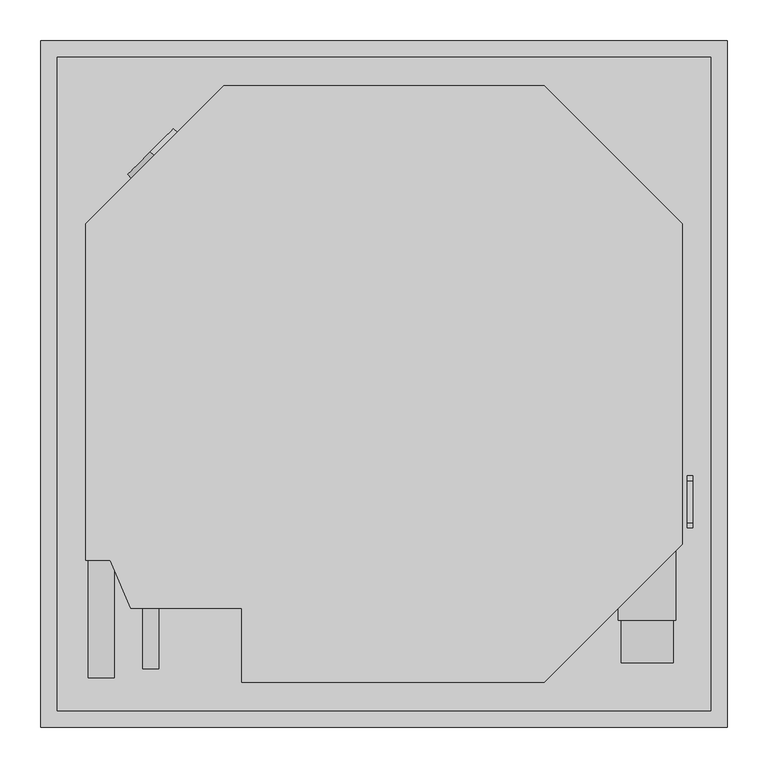
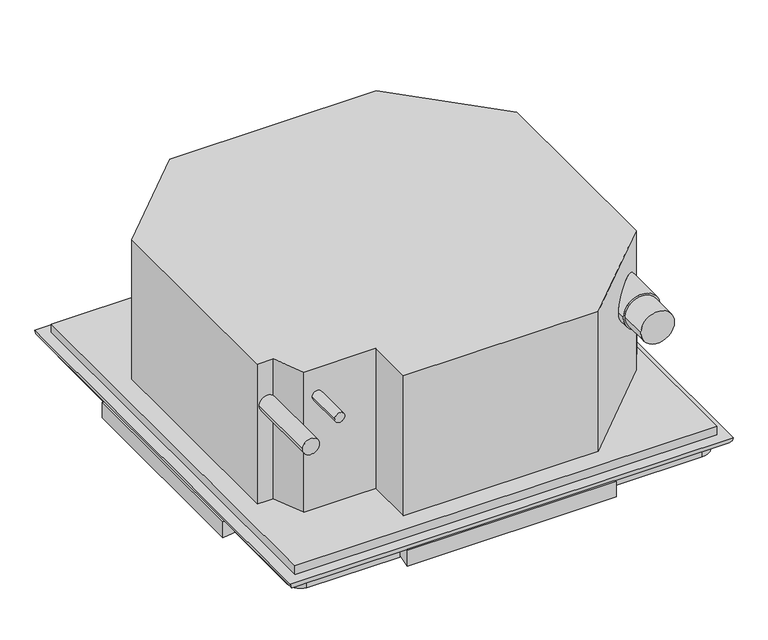
"""IFC4 building model written with IfcOpenShell, lengths in millimetres: proxy geometry, PLFY-P-NBMU-E_4-way_33x33 : PLFY-P36NBMU-E."""

from ifc_helpers import new_model, si_unit, point, frame, frame_2d, origin, place, context, project, spatial, polyline, circle_curve, ellipse_curve, trimmed, segment, composite_curve, outline, extrude, faceted_brep, source, transform, mapped, element, save
from ifc_brep_helpers import plane_surface, cylinder_surface, revolved_surface, advanced_brep


def mechanical_equipment_de7c3da1(model_context):
    return source(origin(), model_context, "Body", "SolidModel", [
        extrude(outline(composite_curve([segment(polyline([(495.9893963, 179.1894012), (433.1276035, 242.0511941), (455.2213333, 399.25625), (626.6713333, 399.25625)]), True, "CONTINUOUS"), segment(trimmed(circle_curve(frame_2d((626.6713333, 372.2612181)), 26.9950319), [point((626.6713333, 399.25625))], [point((653.25625, 376.9488562))], False, "CARTESIAN"), True, "CONTINUOUS"), segment(polyline([(653.25625, 376.9488562), (653.25625, 201.2918161), (495.9893963, 179.1894012)]), True, "CONTINUOUS")], self_intersect=False)), frame((0.0, 0.0, -34.925), z_axis=(0.0, 0.0, 1.0), x_axis=(1.0, 0.0, 0.0)), (0.0, 0.0, 1.0), 25.4),
        extrude(outline(composite_curve([segment(polyline([(495.9893963, -178.4947006), (653.25625, -200.5971155), (653.25625, -376.2541555)]), True, "CONTINUOUS"), segment(trimmed(circle_curve(frame_2d((626.6713333, -371.5665174)), 26.9950319), [point((653.25625, -376.2541555))], [point((626.6713333, -398.5615494))], False, "CARTESIAN"), True, "CONTINUOUS"), segment(polyline([(626.6713333, -398.5615494), (455.2213333, -398.5615494), (433.1276035, -241.3564935), (495.9893963, -178.4947006)]), True, "CONTINUOUS")], self_intersect=False)), frame((0.0, 0.0, -34.925), z_axis=(0.0, 0.0, 1.0), x_axis=(1.0, 0.0, 0.0)), (0.0, 0.0, 1.0), 25.4),
        extrude(outline(composite_curve([segment(polyline([(75.5617928, -241.3), (53.459378, -398.5668537), (-122.1976621, -398.5668537)]), True, "CONTINUOUS"), segment(trimmed(circle_curve(frame_2d((-117.510024, -371.9819369)), 26.9950319), [point((-122.1976621, -398.5668537))], [point((-144.5050559, -371.9819369))], False, "CARTESIAN"), True, "CONTINUOUS"), segment(polyline([(-144.5050559, -371.9819369), (-144.5050559, -200.5319369), (12.7, -178.4382072), (75.5617928, -241.3)]), True, "CONTINUOUS")], self_intersect=False)), frame((0.0, 0.0, -34.925), z_axis=(0.0, 0.0, 1.0), x_axis=(1.0, 0.0, 0.0)), (0.0, 0.0, 1.0), 25.4),
        extrude(outline(composite_curve([segment(polyline([(74.8105988, 242.0202952), (11.9488059, 179.1585024), (-145.25625, 201.2522321), (-145.25625, 372.7022321)]), True, "CONTINUOUS"), segment(trimmed(circle_curve(frame_2d((-118.2612181, 372.7022321)), 26.9950319), [point((-145.25625, 372.7022321))], [point((-122.9488562, 399.2871489))], False, "CARTESIAN"), True, "CONTINUOUS"), segment(polyline([(-122.9488562, 399.2871489), (52.7081839, 399.2871489), (74.8105988, 242.0202952)]), True, "CONTINUOUS")], self_intersect=False)), frame((0.0, 0.0, -34.925), z_axis=(0.0, 0.0, 1.0), x_axis=(1.0, 0.0, 0.0)), (0.0, 0.0, 1.0), 25.4),
        advanced_brep(
        [(657.240471, -403.240471, -16.1614213), (630.124829, -376.124829, -23.2074342), (630.124829, -191.6865644, -23.2074342), (657.240471, -195.4974193, -16.1614213), (630.124829, 376.124829, -23.2074342), (657.240471, 403.240471, -16.1614213), (657.240471, 195.431279, -16.1614213), (630.124829, 191.620424, -23.2074342), (585.0640593, 331.0640593, -30.1625), (618.33125, 189.9629446, -25.2489466), (618.33125, -190.0290849, -25.2489466), (585.0640593, -331.0640593, -30.1625), (495.3, 241.3, 0.0), (495.3, 241.3, -30.1625), (495.3, -241.3, -30.1625), (495.3, -241.3, 0.0), (673.0971264, 419.0971264, 0.0), (673.0971264, -419.0971264, 0.0), (670.1423679, -197.3106627, -9.525), (670.1423679, 197.2445224, -9.525), (449.2705241, -403.240471, -16.1614213), (445.0717378, -376.124829, -23.2074342), (-149.240471, -403.240471, -16.1614213), (-122.124829, -376.124829, -23.2074342), (62.9944025, -376.124829, -23.2074342), (58.7956162, -403.240471, -16.1614213), (444.0290849, -369.3914063, -24.392355), (64.0370554, -369.3914063, -24.392355), (-77.0640593, -331.0640593, -30.1625), (12.7, -241.3, -30.1625), (12.7, -241.3, 0.0), (-165.0971264, -419.0971264, 0.0), (56.7977912, -416.1423679, -9.525), (451.2683492, -416.1423679, -9.525), (-149.240471, -195.431279, -16.1614213), (-122.124829, -191.620424, -23.2074342), (-149.240471, 403.240471, -16.1614213), (-122.124829, 376.124829, -23.2074342), (-122.124829, 191.6865644, -23.2074342), (-149.240471, 195.4974193, -16.1614213), (-110.33125, -189.9629446, -25.2489466), (-110.33125, 190.0290849, -25.2489466), (-77.0640593, 331.0640593, -30.1625), (12.7, 241.3, -30.1625), (12.7, 241.3, 0.0), (-165.0971264, 419.0971264, 0.0), (-162.1423679, 197.3106627, -9.525), (-162.1423679, -197.2445224, -9.525), (58.5025807, 403.240471, -16.1614213), (62.3134356, 376.124829, -23.2074342), (445.620424, 376.124829, -23.2074342), (449.431279, 403.240471, -16.1614213), (63.9709151, 364.33125, -25.2489466), (443.9629446, 364.33125, -25.2489466), (451.2445224, 416.1423679, -9.525), (56.6893373, 416.1423679, -9.525), (56.3398096, -419.1, -9.525), (451.7263308, -419.1, -9.525), (451.7263308, -419.1, -41.275), (56.3398096, -419.1, -41.275), (64.0370554, -369.3914063, -41.275), (444.0290849, -369.3914063, -41.275), (673.1, -197.7263308, -9.525), (673.1, 197.6601904, -9.525), (673.1, -197.7263308, -41.275), (618.33125, -190.0290849, -41.275), (618.33125, 189.9629446, -41.275), (673.1, 197.6601904, -41.275), (451.6601904, 419.1, -9.525), (56.2736692, 419.1, -9.525), (56.2736692, 419.1, -41.275), (451.6601904, 419.1, -41.275), (443.9629446, 364.33125, -41.275), (63.9709151, 364.33125, -41.275), (-165.1, 197.7263308, -9.525), (-165.1, -197.6601904, -9.525), (-165.1, 197.7263308, -41.275), (-110.33125, 190.0290849, -41.275), (-110.33125, -189.9629446, -41.275), (-165.1, -197.6601904, -41.275)],
        [
            (0, 1, ellipse_curve(frame((657.240471, -403.240471, -71.8598951), z_axis=(-0.7071067811865475, -0.7071067811865475, 0.0), x_axis=(0.7071067811865474, -0.7071067811865476, 0.0)), 78.7695371, 55.6984738)),
            (1, 2),
            (2, 3, ellipse_curve(frame((657.240471, -195.4974193, -71.8598951), z_axis=(0.13917310096006688, 0.9902680687415701, 0.0), x_axis=(0.9902680687415703, -0.1391731009600663, 0.0)), 56.2458546, 55.6984738)),
            (3, 0),
            (4, 5, ellipse_curve(frame((657.240471, 403.240471, -71.8598951), z_axis=(-0.7071067811865475, 0.7071067811865475, 0.0), x_axis=(-0.7071067811865474, -0.7071067811865476, 0.0)), 78.7695371, 55.6984738)),
            (5, 6),
            (6, 7, ellipse_curve(frame((657.240471, 195.431279, -71.8598951), z_axis=(0.13917310096006905, -0.9902680687415698, 0.0), x_axis=(-0.9902680687415699, -0.13917310096006894, 0.0)), 56.2458546, 55.6984738)),
            (7, 4),
            (8, 4, ellipse_curve(frame((467.2055779, 213.2055779, 882.8722668), z_axis=(0.7071067811865475, -0.7071067811865475, 0.0), x_axis=(0.7071067811865474, 0.7071067811865476, 0.0)), 1301.9394049, 920.6101819)),
            (7, 9, ellipse_curve(frame((467.2055779, 168.7236165, 882.8722668), z_axis=(-0.13917310096006905, 0.9902680687415698, 0.0), x_axis=(0.9902680687415699, 0.13917310096006894, 0.0)), 929.6575452, 920.6101819)),
            (9, 10),
            (10, 2, ellipse_curve(frame((467.2055779, -168.7897568, 882.8722668), z_axis=(-0.13917310096006688, -0.9902680687415701, 0.0), x_axis=(-0.9902680687415703, 0.1391731009600663, 0.0)), 929.6575452, 920.6101819)),
            (1, 11, ellipse_curve(frame((467.2055779, -213.2055779, 882.8722668), z_axis=(0.7071067811865475, 0.7071067811865475, 0.0), x_axis=(-0.7071067811865474, 0.7071067811865476, 0.0)), 1301.9394049, 920.6101819)),
            (11, 8),
            (12, 13),
            (13, 14),
            (14, 15),
            (15, 12),
            (5, 16, ellipse_curve(frame((657.240471, 403.240471, -0.3018923), z_axis=(0.7071067811865475, -0.7071067811865475, 0.0), x_axis=(0.7071067811865474, 0.7071067811865476, 0.0)), 22.428761, 15.859529)),
            (16, 17),
            (17, 0, ellipse_curve(frame((657.240471, -403.240471, -0.3018923), z_axis=(0.7071067811865475, 0.7071067811865475, 0.0), x_axis=(-0.7071067811865474, 0.7071067811865476, 0.0)), 22.428761, 15.859529)),
            (3, 18, ellipse_curve(frame((657.240471, -195.4974193, -0.3018923), z_axis=(-0.13917310096006688, -0.9902680687415701, 0.0), x_axis=(-0.9902680687415703, 0.1391731009600663, 0.0)), 16.0153897, 15.859529)),
            (18, 19),
            (19, 6, ellipse_curve(frame((657.240471, 195.431279, -0.3018923), z_axis=(-0.13917310096006905, 0.9902680687415698, 0.0), x_axis=(0.9902680687415699, 0.13917310096006894, 0.0)), 16.0153897, 15.859529)),
            (0, 20),
            (20, 21, ellipse_curve(frame((449.2705241, -403.240471, -71.8598951), z_axis=(-0.9882225229323841, -0.15302367519163051, 0.0), x_axis=(-0.1530236751916298, 0.9882225229323841, 0.0)), 56.3622793, 55.6984738)),
            (21, 1),
            (22, 23, ellipse_curve(frame((-149.240471, -403.240471, -71.8598951), z_axis=(-0.7071067811865475, 0.7071067811865475, 0.0), x_axis=(-0.7071067811865476, -0.7071067811865474, 0.0)), 78.7695371, 55.6984738)),
            (23, 24),
            (24, 25, ellipse_curve(frame((58.7956162, -403.240471, -71.8598951), z_axis=(0.9882225229323951, -0.15302367519155985, 0.0), x_axis=(-0.153023675191559, -0.9882225229323952, 0.0)), 56.3622793, 55.6984738)),
            (25, 22),
            (21, 26, ellipse_curve(frame((419.8441176, -213.2055779, 882.8722668), z_axis=(0.9882225229323841, 0.15302367519163051, 0.0), x_axis=(0.1530236751916298, -0.9882225229323841, 0.0)), 931.5818659, 920.6101819)),
            (26, 27),
            (27, 24, ellipse_curve(frame((88.2220228, -213.2055779, 882.8722668), z_axis=(-0.9882225229323951, 0.15302367519155985, 0.0), x_axis=(0.153023675191559, 0.9882225229323952, 0.0)), 931.5818659, 920.6101819)),
            (23, 28, ellipse_curve(frame((40.7944221, -213.2055779, 882.8722668), z_axis=(0.7071067811865475, -0.7071067811865475, 0.0), x_axis=(0.7071067811865476, 0.7071067811865474, 0.0)), 1301.9394049, 920.6101819)),
            (28, 11),
            (14, 29),
            (29, 30),
            (30, 15),
            (17, 31),
            (31, 22, ellipse_curve(frame((-149.240471, -403.240471, -0.3018923), z_axis=(0.7071067811865475, -0.7071067811865475, 0.0), x_axis=(0.7071067811865476, 0.7071067811865474, 0.0)), 22.428761, 15.859529)),
            (25, 32, ellipse_curve(frame((58.7956162, -403.240471, -0.3018923), z_axis=(-0.9882225229323951, 0.15302367519155985, 0.0), x_axis=(0.153023675191559, 0.9882225229323952, 0.0)), 16.0485403, 15.859529)),
            (32, 33),
            (33, 20, ellipse_curve(frame((449.2705241, -403.240471, -0.3018923), z_axis=(0.9882225229323841, 0.15302367519163051, 0.0), x_axis=(0.1530236751916298, -0.9882225229323841, 0.0)), 16.0485403, 15.859529)),
            (22, 34),
            (34, 35, ellipse_curve(frame((-149.240471, -195.431279, -71.8598951), z_axis=(-0.13917310096007277, 0.9902680687415694, 0.0), x_axis=(0.9902680687415695, 0.13917310096007157, 0.0)), 56.2458546, 55.6984738)),
            (35, 23),
            (36, 37, ellipse_curve(frame((-149.240471, 403.240471, -71.8598951), z_axis=(0.7071067811865475, 0.7071067811865475, 0.0), x_axis=(-0.7071067811865474, 0.7071067811865476, 0.0)), 78.7695371, 55.6984738)),
            (37, 38),
            (38, 39, ellipse_curve(frame((-149.240471, 195.4974193, -71.8598951), z_axis=(-0.13917310096006336, -0.9902680687415706, 0.0), x_axis=(-0.9902680687415705, 0.1391731009600634, 0.0)), 56.2458546, 55.6984738)),
            (39, 36),
            (35, 40, ellipse_curve(frame((40.7944221, -168.7236165, 882.8722668), z_axis=(0.13917310096007277, -0.9902680687415694, 0.0), x_axis=(-0.9902680687415695, -0.13917310096007157, 0.0)), 929.6575452, 920.6101819)),
            (40, 41),
            (41, 38, ellipse_curve(frame((40.7944221, 168.7897568, 882.8722668), z_axis=(0.13917310096006336, 0.9902680687415706, 0.0), x_axis=(0.9902680687415705, -0.1391731009600634, 0.0)), 929.6575452, 920.6101819)),
            (37, 42, ellipse_curve(frame((40.7944221, 213.2055779, 882.8722668), z_axis=(-0.7071067811865475, -0.7071067811865475, 0.0), x_axis=(0.7071067811865474, -0.7071067811865476, 0.0)), 1301.9394049, 920.6101819)),
            (42, 28),
            (29, 43),
            (43, 44),
            (44, 30),
            (31, 45),
            (45, 36, ellipse_curve(frame((-149.240471, 403.240471, -0.3018923), z_axis=(-0.7071067811865475, -0.7071067811865475, 0.0), x_axis=(0.7071067811865474, -0.7071067811865476, 0.0)), 22.428761, 15.859529)),
            (39, 46, ellipse_curve(frame((-149.240471, 195.4974193, -0.3018923), z_axis=(0.13917310096006336, 0.9902680687415706, 0.0), x_axis=(0.9902680687415705, -0.1391731009600634, 0.0)), 16.0153897, 15.859529)),
            (46, 47),
            (47, 34, ellipse_curve(frame((-149.240471, -195.431279, -0.3018923), z_axis=(0.13917310096007277, -0.9902680687415694, 0.0), x_axis=(-0.9902680687415695, -0.13917310096007157, 0.0)), 16.0153897, 15.859529)),
            (36, 48),
            (48, 49, ellipse_curve(frame((58.5025807, 403.240471, -71.8598951), z_axis=(0.9902680687415706, 0.13917310096006327, 0.0), x_axis=(0.1391731009600635, -0.9902680687415705, 0.0)), 56.2458546, 55.6984738)),
            (49, 37),
            (4, 50),
            (50, 51, ellipse_curve(frame((449.431279, 403.240471, -71.8598951), z_axis=(-0.9902680687415695, 0.13917310096007188, 0.0), x_axis=(0.13917310096007085, 0.9902680687415695, 0.0)), 56.2458546, 55.6984738)),
            (51, 5),
            (8, 42),
            (49, 52, ellipse_curve(frame((85.2102432, 213.2055779, 882.8722668), z_axis=(-0.9902680687415706, -0.13917310096006327, 0.0), x_axis=(-0.1391731009600635, 0.9902680687415705, 0.0)), 929.6575452, 920.6101819)),
            (52, 53),
            (53, 50, ellipse_curve(frame((422.7236165, 213.2055779, 882.8722668), z_axis=(0.9902680687415695, -0.13917310096007188, 0.0), x_axis=(-0.13917310096007085, -0.9902680687415695, 0.0)), 929.6575452, 920.6101819)),
            (13, 43),
            (12, 44),
            (16, 45),
            (51, 54, ellipse_curve(frame((449.431279, 403.240471, -0.3018923), z_axis=(0.9902680687415695, -0.13917310096007188, 0.0), x_axis=(-0.13917310096007085, -0.9902680687415695, 0.0)), 16.0153897, 15.859529)),
            (54, 55),
            (55, 48, ellipse_curve(frame((58.5025807, 403.240471, -0.3018923), z_axis=(-0.9902680687415706, -0.13917310096006327, 0.0), x_axis=(-0.1391731009600635, 0.9902680687415705, 0.0)), 16.0153897, 15.859529)),
            (56, 57),
            (57, 33),
            (32, 56),
            (58, 59),
            (59, 60),
            (60, 61),
            (61, 58),
            (61, 26),
            (57, 58),
            (60, 27),
            (59, 56),
            (62, 63),
            (63, 19),
            (18, 62),
            (64, 65),
            (65, 66),
            (66, 67),
            (67, 64),
            (62, 64),
            (67, 63),
            (66, 9),
            (65, 10),
            (68, 69),
            (69, 55),
            (54, 68),
            (70, 71),
            (71, 72),
            (72, 73),
            (73, 70),
            (73, 52),
            (69, 70),
            (72, 53),
            (71, 68),
            (74, 75),
            (75, 47),
            (46, 74),
            (76, 77),
            (77, 78),
            (78, 79),
            (79, 76),
            (74, 76),
            (79, 75),
            (78, 40),
            (77, 41),
        ],
        [
            revolved_surface(polyline([(712.9389448, -458.9389448343353, -71.8598951), (712.9389448, -187.6695092991689, -71.8598951)]), (657.240471, 419.1, -71.8598951), (0.0, -1.0, 0.0)),
            revolved_surface(polyline([(712.9389448, 187.60336899916882, -71.8598951), (712.9389448, 458.93894483433536, -71.8598951)]), (657.240471, 419.1, -71.8598951), (0.0, -1.0, 0.0)),
            cylinder_surface(frame((467.2055779, 419.1, 882.8722668), z_axis=(0.0, 1.0, 0.0), x_axis=(1.0, 0.0, 0.0)), 920.6101819),
            plane_surface(frame((495.3, 241.3, -30.1625), z_axis=(-1.0, 0.0, 0.0), x_axis=(0.0, -1.0, 0.0))),
            cylinder_surface(frame((657.240471, 419.1, -0.3018923), z_axis=(0.0, 1.0, 0.0), x_axis=(1.0, 0.0, 0.0)), 15.859529),
            revolved_surface(polyline([(440.64576097933684, -458.9389448, -71.8598951), (712.9389448343353, -458.9389448, -71.8598951)]), (673.1, -403.240471, -71.8598951), (-1.0, 0.0, 0.0)),
            revolved_surface(polyline([(-204.9389448343353, -458.9389448, -71.8598951), (67.42037932065921, -458.9389448, -71.8598951)]), (673.1, -403.240471, -71.8598951), (-1.0, 0.0, 0.0)),
            cylinder_surface(frame((673.1, -213.2055779, 882.8722668), z_axis=(1.0, 0.0, 0.0), x_axis=(0.0, -1.0, 0.0)), 920.6101819),
            plane_surface(frame((495.3, -241.3, -30.1625), z_axis=(0.0, 1.0, 0.0), x_axis=(-1.0, 0.0, 0.0))),
            cylinder_surface(frame((673.1, -403.240471, -0.3018923), z_axis=(1.0, 0.0, 0.0), x_axis=(0.0, -1.0, 0.0)), 15.859529),
            revolved_surface(polyline([(-204.9389448, -187.60336899916868, -71.8598951), (-204.9389448, -458.9389448343353, -71.8598951)]), (-149.240471, -419.1, -71.8598951), (0.0, 1.0, 0.0)),
            revolved_surface(polyline([(-204.9389448, 458.9389448343353, -71.8598951), (-204.9389448, 187.66950929916914, -71.8598951)]), (-149.240471, -419.1, -71.8598951), (0.0, 1.0, 0.0)),
            cylinder_surface(frame((40.7944221, -419.1, 882.8722668), z_axis=(0.0, -1.0, 0.0), x_axis=(-1.0, 0.0, 0.0)), 920.6101819),
            plane_surface(frame((12.7, -241.3, -30.1625), z_axis=(1.0, 0.0, 0.0), x_axis=(0.0, 1.0, 0.0))),
            cylinder_surface(frame((-149.240471, -419.1, -0.3018923), z_axis=(0.0, -1.0, 0.0), x_axis=(-1.0, 0.0, 0.0)), 15.859529),
            revolved_surface(polyline([(66.33049070083086, 458.9389448, -71.8598951), (-204.93894483433533, 458.9389448, -71.8598951)]), (-165.1, 403.240471, -71.8598951), (1.0, 0.0, 0.0)),
            revolved_surface(polyline([(712.9389448343353, 458.9389448, -71.8598951), (441.60336899916877, 458.9389448, -71.8598951)]), (-165.1, 403.240471, -71.8598951), (1.0, 0.0, 0.0)),
            cylinder_surface(frame((-165.1, 213.2055779, 882.8722668), z_axis=(-1.0, 0.0, 0.0), x_axis=(0.0, 1.0, 0.0)), 920.6101819),
            plane_surface(frame((-77.0640593, 331.0640593, -30.1625), z_axis=(0.0, 0.0, -1.0), x_axis=(1.0, 0.0, 0.0))),
            plane_surface(frame((12.7, 241.3, -30.1625), z_axis=(0.0, -1.0, 0.0), x_axis=(1.0, 0.0, 0.0))),
            plane_surface(frame((12.7, 241.3, 0.0), z_axis=(0.0, 0.0, 1.0), x_axis=(1.0, 0.0, 0.0))),
            cylinder_surface(frame((-165.1, 403.240471, -0.3018923), z_axis=(-1.0, 0.0, 0.0), x_axis=(0.0, 1.0, 0.0)), 15.859529),
            plane_surface(frame((444.0290849, -369.3914063, -9.525), z_axis=(0.0, 0.0, 1.0), x_axis=(-0.15302367519163051, 0.9882225229323841, 0.0))),
            plane_surface(frame((444.0290849, -369.3914063, -41.275), z_axis=(0.0, 0.0, -1.0), x_axis=(0.15302367519163051, -0.9882225229323841, 0.0))),
            plane_surface(frame((451.7263308, -419.1, -9.525), z_axis=(0.9882225229323841, 0.15302367519163051, 0.0), x_axis=(0.0, 0.0, -1.0))),
            plane_surface(frame((444.0290849, -369.3914063, -9.525), z_axis=(0.0, 1.0, 0.0), x_axis=(0.0, 0.0, -1.0))),
            plane_surface(frame((64.0370554, -369.3914063, -9.525), z_axis=(-0.9882225229323951, 0.15302367519155985, 0.0), x_axis=(0.0, 0.0, -1.0))),
            plane_surface(frame((56.3398096, -419.1, -9.525), z_axis=(0.0, -1.0, 0.0), x_axis=(0.0, 0.0, -1.0))),
            plane_surface(frame((673.1, -988.0353065, -9.525), z_axis=(0.0, 0.0, 1.0), x_axis=(0.0, 1.0, 0.0))),
            plane_surface(frame((673.1, -988.0353065, -41.275), z_axis=(0.0, 0.0, -1.0), x_axis=(0.0, -1.0, 0.0))),
            plane_surface(frame((673.1, -197.7263308, -9.525), z_axis=(1.0, 0.0, 0.0), x_axis=(0.0, 0.0, -1.0))),
            plane_surface(frame((673.1, 197.6601904, -9.525), z_axis=(-0.13917310096006905, 0.9902680687415698, 0.0), x_axis=(0.0, 0.0, -1.0))),
            plane_surface(frame((618.33125, 189.9629446, -9.525), z_axis=(-1.0, 0.0, 0.0), x_axis=(0.0, 0.0, -1.0))),
            plane_surface(frame((618.33125, -190.0290849, -9.525), z_axis=(-0.13917310096006688, -0.9902680687415701, 0.0), x_axis=(0.0, 0.0, -1.0))),
            plane_surface(frame((81.1605988, 242.0202952, -9.525), z_axis=(0.0, 0.0, 1.0), x_axis=(0.13917310096006327, -0.9902680687415706, 0.0))),
            plane_surface(frame((81.1605988, 242.0202952, -41.275), z_axis=(0.0, 0.0, -1.0), x_axis=(-0.13917310096006327, 0.9902680687415706, 0.0))),
            plane_surface(frame((56.2736692, 419.1, -9.525), z_axis=(-0.9902680687415706, -0.13917310096006327, 0.0), x_axis=(0.0, 0.0, -1.0))),
            plane_surface(frame((63.9709151, 364.33125, -9.525), z_axis=(0.0, -1.0, 0.0), x_axis=(0.0, 0.0, -1.0))),
            plane_surface(frame((443.9629446, 364.33125, -9.525), z_axis=(0.9902680687415695, -0.13917310096007188, 0.0), x_axis=(0.0, 0.0, -1.0))),
            plane_surface(frame((451.6601904, 419.1, -9.525), z_axis=(0.0, 1.0, 0.0), x_axis=(0.0, 0.0, -1.0))),
            plane_surface(frame((-165.1, 988.0353065, -9.525), z_axis=(0.0, 0.0, 1.0), x_axis=(0.0, -1.0, 0.0))),
            plane_surface(frame((-165.1, 988.0353065, -41.275), z_axis=(0.0, 0.0, -1.0), x_axis=(0.0, 1.0, 0.0))),
            plane_surface(frame((-165.1, 197.7263308, -9.525), z_axis=(-1.0, 0.0, 0.0), x_axis=(0.0, 0.0, -1.0))),
            plane_surface(frame((-165.1, -197.6601904, -9.525), z_axis=(0.13917310096007277, -0.9902680687415694, 0.0), x_axis=(0.0, 0.0, -1.0))),
            plane_surface(frame((-110.33125, -189.9629446, -9.525), z_axis=(1.0, 0.0, 0.0), x_axis=(0.0, 0.0, -1.0))),
            plane_surface(frame((-110.33125, 190.0290849, -9.525), z_axis=(0.13917310096006336, 0.9902680687415706, 0.0), x_axis=(0.0, 0.0, -1.0))),
        ],
        [
            (0, [[1, 2, 3, 4]]),
            (1, [[5, 6, 7, 8]]),
            (2, [[9, -8, 10, 11, 12, -2, 13, 14]]),
            (3, [[15, 16, 17, 18]]),
            (4, [[19, 20, 21, -4, 22, 23, 24, -6]]),
            (5, [[-1, 25, 26, 27]]),
            (6, [[28, 29, 30, 31]]),
            (7, [[-13, -27, 32, 33, 34, -29, 35, 36]]),
            (8, [[-17, 37, 38, 39]]),
            (9, [[-21, 40, 41, -31, 42, 43, 44, -25]]),
            (10, [[-28, 45, 46, 47]]),
            (11, [[48, 49, 50, 51]]),
            (12, [[-35, -47, 52, 53, 54, -49, 55, 56]]),
            (13, [[-38, 57, 58, 59]]),
            (14, [[-41, 60, 61, -51, 62, 63, 64, -45]]),
            (15, [[-48, 65, 66, 67]]),
            (16, [[-5, 68, 69, 70]]),
            (17, [[-9, 71, -55, -67, 72, 73, 74, -68]]),
            (18, [[-14, -36, -56, -71], [-16, 75, -57, -37]]),
            (19, [[-15, 76, -58, -75]]),
            (20, [[-20, 77, -60, -40], [-18, -39, -59, -76]]),
            (21, [[-19, -70, 78, 79, 80, -65, -61, -77]]),
            (22, [[81, 82, -43, 83]]),
            (23, [[84, 85, 86, 87]]),
            (24, [[-87, 88, -32, -26, -44, -82, 89]]),
            (25, [[-86, 90, -33, -88]]),
            (26, [[-85, 91, -83, -42, -30, -34, -90]]),
            (27, [[-81, -91, -84, -89]]),
            (28, [[92, 93, -23, 94]]),
            (29, [[95, 96, 97, 98]]),
            (30, [[-92, 99, -98, 100]]),
            (31, [[-97, 101, -10, -7, -24, -93, -100]]),
            (32, [[-96, 102, -11, -101]]),
            (33, [[-95, -99, -94, -22, -3, -12, -102]]),
            (34, [[103, 104, -79, 105]]),
            (35, [[106, 107, 108, 109]]),
            (36, [[-109, 110, -72, -66, -80, -104, 111]]),
            (37, [[-108, 112, -73, -110]]),
            (38, [[-107, 113, -105, -78, -69, -74, -112]]),
            (39, [[-103, -113, -106, -111]]),
            (40, [[114, 115, -63, 116]]),
            (41, [[117, 118, 119, 120]]),
            (42, [[-114, 121, -120, 122]]),
            (43, [[-119, 123, -52, -46, -64, -115, -122]]),
            (44, [[-118, 124, -53, -123]]),
            (45, [[-117, -121, -116, -62, -50, -54, -124]]),
        ],
    ),
        faceted_brep([(-145.25625, 399.25625, 17.4625), (-145.25625, -399.25625, 17.4625), (653.25625, -399.25625, 17.4625), (653.25625, 399.25625, 17.4625), (-145.25625, 399.25625, 0.0), (653.25625, 399.25625, 0.0), (653.25625, -399.25625, 0.0), (-145.25625, -399.25625, 0.0), (-37.597716, -314.3813928, 0.0), (545.597716, -314.3813928, 0.0), (545.597716, 285.5943885, 0.0), (-37.597716, 285.5943885, 0.0), (-37.597716, 285.5943885, -9.525), (545.597716, 285.5943885, -9.525), (545.597716, -314.3813928, -9.525), (-37.597716, -314.3813928, -9.525)], [[[0, 1, 2, 3]], [[4, 5, 6, 7], [8, 9, 10, 11]], [[1, 0, 4, 7]], [[2, 1, 7, 6]], [[3, 2, 6, 5]], [[0, 3, 5, 4]], [[12, 13, 14, 15]], [[12, 15, 8, 11]], [[15, 14, 9, 8]], [[14, 13, 10, 9]], [[13, 12, 11, 10]]]),
        advanced_brep(
        [(449.7291217, 364.33125, 297.9539062), (58.2708783, 364.33125, 297.9539062), (-110.33125, 195.7291217, 297.9539062), (-110.33125, -215.4259931, 297.9539062), (-80.4797249, -215.4259931, 297.9539062), (-55.6682982, -273.8780513, 297.9539062), (80.398975, -273.8780513, 297.9539062), (80.398975, -364.33125, 297.9539062), (449.7291217, -364.33125, 297.9539062), (618.33125, -195.7291217, 297.9539062), (618.33125, 195.7291217, 297.9539062), (449.7291217, 364.33125, 17.4625), (618.33125, 195.7291217, 17.4625), (618.33125, -195.7291217, 17.4625), (449.7291217, -364.33125, 17.4625), (80.398975, -364.33125, 17.4625), (80.398975, -273.8780513, 17.4625), (-55.6682982, -273.8780513, 17.4625), (-80.4797249, -215.4259931, 17.4625), (-110.33125, -215.4259931, 17.4625), (-110.33125, 195.7291217, 17.4625), (58.2708783, 364.33125, 17.4625), (610.4929688, -203.567403, 207.16875), (540.4445313, -273.6158405, 207.16875), (540.4445313, -288.528125, 207.16875), (610.4929688, -288.528125, 207.16875)],
        [
            (0, 1),
            (1, 2),
            (2, 3),
            (3, 4),
            (4, 5),
            (5, 6),
            (6, 7),
            (7, 8),
            (8, 9),
            (9, 10),
            (10, 0),
            (11, 12),
            (12, 13),
            (13, 14),
            (14, 15),
            (15, 16),
            (16, 17),
            (17, 18),
            (18, 19),
            (19, 20),
            (20, 21),
            (21, 11),
            (0, 11),
            (21, 1),
            (20, 2),
            (19, 3),
            (18, 4),
            (17, 5),
            (16, 6),
            (15, 7),
            (14, 8),
            (13, 9),
            (22, 23, ellipse_curve(frame((575.46875, -238.5916217, 207.16875), z_axis=(-0.7071067811865432, 0.7071067811865518, 0.0), x_axis=(-0.7071067811865518, -0.7071067811865434, 0.0)), 49.5317252, 35.0242188)),
            (23, 22, ellipse_curve(frame((575.46875, -238.5916217, 207.16875), z_axis=(-0.7071067811865432, 0.7071067811865518, 0.0), x_axis=(-0.7071067811865518, -0.7071067811865434, 0.0)), 49.5317252, 35.0242188)),
            (12, 10),
            (24, 25, circle_curve(frame((575.46875, -288.528125, 207.16875), z_axis=(0.0, -1.0, 0.0), x_axis=(0.0, 0.0, 1.0)), 35.0242188)),
            (25, 24, circle_curve(frame((575.46875, -288.528125, 207.16875), z_axis=(0.0, -1.0, 0.0), x_axis=(0.0, 0.0, 1.0)), 35.0242187)),
            (24, 23),
            (22, 25),
        ],
        [
            plane_surface(frame((58.2708783, 364.33125, 297.9539062), z_axis=(0.0, 0.0, 1.0), x_axis=(-1.0, 0.0, 0.0))),
            plane_surface(frame((58.2708783, 364.33125, 17.4625), z_axis=(0.0, 0.0, -1.0), x_axis=(1.0, 0.0, 0.0))),
            plane_surface(frame((449.7291217, 364.33125, 297.9539062), z_axis=(0.0, 1.0, 0.0), x_axis=(0.0, 0.0, -1.0))),
            plane_surface(frame((58.2708783, 364.33125, 297.9539062), z_axis=(-0.7071067811865495, 0.7071067811865456, 0.0), x_axis=(0.0, 0.0, -1.0))),
            plane_surface(frame((-110.33125, 195.7291217, 297.9539062), z_axis=(-1.0, 0.0, 0.0), x_axis=(0.0, 0.0, -1.0))),
            plane_surface(frame((-110.33125, -215.4259931, 297.9539062), z_axis=(0.0, -1.0, 0.0), x_axis=(0.0, 0.0, -1.0))),
            plane_surface(frame((-80.4797249, -215.4259931, 297.9539062), z_axis=(-0.9205048534524416, -0.390731128489271, 0.0), x_axis=(0.0, 0.0, -1.0))),
            plane_surface(frame((-55.6682982, -273.8780513, 297.9539062), z_axis=(0.0, -1.0, 0.0), x_axis=(0.0, 0.0, -1.0))),
            plane_surface(frame((80.398975, -273.8780513, 297.9539062), z_axis=(-1.0, 0.0, 0.0), x_axis=(0.0, 0.0, -1.0))),
            plane_surface(frame((80.398975, -364.33125, 297.9539062), z_axis=(0.0, -1.0, 0.0), x_axis=(0.0, 0.0, -1.0))),
            plane_surface(frame((449.7291217, -364.33125, 297.9539062), z_axis=(0.7071067811865432, -0.7071067811865518, 0.0), x_axis=(0.0, 0.0, -1.0))),
            plane_surface(frame((618.33125, -195.7291217, 297.9539062), z_axis=(1.0, 0.0, 0.0), x_axis=(0.0, 0.0, -1.0))),
            plane_surface(frame((618.33125, 195.7291217, 297.9539062), z_axis=(0.7071067811865456, 0.7071067811865497, 0.0), x_axis=(0.0, 0.0, -1.0))),
            plane_surface(frame((575.46875, -288.528125, 242.1929687), z_axis=(0.0, -1.0, 0.0), x_axis=(-1.0, 0.0, 0.0))),
            cylinder_surface(frame((575.46875, -178.4947006, 207.16875), z_axis=(0.0, -1.0, 0.0), x_axis=(0.0, 0.0, 1.0)), 35.0242188),
        ],
        [
            (0, [[1, 2, 3, 4, 5, 6, 7, 8, 9, 10, 11]]),
            (1, [[12, 13, 14, 15, 16, 17, 18, 19, 20, 21, 22]]),
            (2, [[-1, 23, -22, 24]]),
            (3, [[-2, -24, -21, 25]]),
            (4, [[-3, -25, -20, 26]]),
            (5, [[-4, -26, -19, 27]]),
            (6, [[-5, -27, -18, 28]]),
            (7, [[-6, -28, -17, 29]]),
            (8, [[-7, -29, -16, 30]]),
            (9, [[-8, -30, -15, 31]]),
            (10, [[-9, -31, -14, 32], [33, 34]]),
            (11, [[-10, -32, -13, 35]]),
            (12, [[-11, -35, -12, -23]]),
            (13, [[36, 37]]),
            (14, [[-36, 38, -33, 39]]),
            (14, [[-37, -39, -34, -38]]),
        ],
    ),
        extrude(outline(composite_curve([segment(trimmed(circle_curve(frame_2d((207.16875, 575.46875)), 31.8492188), [point((207.16875, 543.6195313))], [point((207.16875, 607.3179688))], False, "CARTESIAN"), True, "CONTINUOUS"), segment(trimmed(circle_curve(frame_2d((207.16875, 575.46875)), 31.8492188), [point((207.16875, 607.3179688))], [point((207.16875, 543.6195313))], False, "CARTESIAN"), True, "CONTINUOUS")], self_intersect=False)), frame((0.0, -340.51875, 0.0), z_axis=(0.0, 1.0, 0.0), x_axis=(0.0, 0.0, 1.0)), (0.0, 0.0, 1.0), 51.990625),
        extrude(outline(composite_curve([segment(trimmed(circle_curve(frame_2d((0.0, -39.5882812)), 39.5882813), [point((0.0, -79.1765625))], [point((0.0, 0.0))], False, "CARTESIAN"), True, "CONTINUOUS"), segment(trimmed(circle_curve(frame_2d((0.0, -39.5882812)), 39.5882813), [point((0.0, 0.0))], [point((0.0, -79.1765625))], False, "CARTESIAN"), True, "CONTINUOUS")], self_intersect=False)), frame((-26.7609219, 279.2994499, 138.1125), z_axis=(-0.7071067811865495, 0.7071067811865456, 0.0), x_axis=(0.7071067811865456, 0.7071067811865495, 0.0)), (0.0, 0.0, 1.0), 6.35),
        extrude(outline(composite_curve([segment(trimmed(circle_curve(frame_2d((213.51875, -91.28125)), 15.875), [point((213.51875, -107.15625))], [point((213.51875, -75.40625))], False, "CARTESIAN"), True, "CONTINUOUS"), segment(trimmed(circle_curve(frame_2d((213.51875, -91.28125)), 15.875), [point((213.51875, -75.40625))], [point((213.51875, -107.15625))], False, "CARTESIAN"), True, "CONTINUOUS")], self_intersect=False)), frame((0.0, -358.9085201, 0.0), z_axis=(0.0, 1.0, 0.0), x_axis=(0.0, 0.0, 1.0)), (0.0, 0.0, 1.0), 143.4825269),
        extrude(outline(composite_curve([segment(trimmed(circle_curve(frame_2d((243.68125, -30.95625)), 9.525), [point((243.68125, -40.48125))], [point((243.68125, -21.43125))], False, "CARTESIAN"), True, "CONTINUOUS"), segment(trimmed(circle_curve(frame_2d((243.68125, -30.95625)), 9.525), [point((243.68125, -21.43125))], [point((243.68125, -40.48125))], False, "CARTESIAN"), True, "CONTINUOUS")], self_intersect=False)), frame((0.0, -347.8952388, 0.0), z_axis=(0.0, 1.0, 0.0), x_axis=(0.0, 0.0, 1.0)), (0.0, 0.0, 1.0), 74.0171875),
        extrude(outline(composite_curve([segment(trimmed(circle_curve(frame_2d((207.16875, 575.46875)), 31.8492188), [point((207.16875, 543.6195313))], [point((207.16875, 607.3179688))], False, "CARTESIAN"), True, "CONTINUOUS"), segment(trimmed(circle_curve(frame_2d((207.16875, 575.46875)), 31.8492188), [point((207.16875, 607.3179688))], [point((207.16875, 543.6195313))], False, "CARTESIAN"), True, "CONTINUOUS")], self_intersect=False)), frame((0.0, -340.51875, 0.0), z_axis=(0.0, 1.0, 0.0), x_axis=(0.0, 0.0, 1.0)), (0.0, 0.0, 1.0), 51.990625),
        extrude(outline(composite_curve([segment(trimmed(circle_curve(frame_2d((-118.7050999, 74.647381)), 6.35), [point((-118.7050999, 80.997381))], [point((-112.3550999, 74.647381))], False, "CARTESIAN"), True, "CONTINUOUS"), segment(polyline([(-112.3550999, 74.647381), (-112.3550999, 36.547381)]), True, "CONTINUOUS"), segment(trimmed(circle_curve(frame_2d((-118.7050999, 36.547381)), 6.35), [point((-112.3550999, 36.547381))], [point((-118.7050999, 30.197381))], False, "CARTESIAN"), True, "CONTINUOUS"), segment(polyline([(-118.7050999, 30.197381), (-169.5050999, 30.197381)]), True, "CONTINUOUS"), segment(trimmed(circle_curve(frame_2d((-169.5050999, 36.547381)), 6.35), [point((-169.5050999, 30.197381))], [point((-175.8550999, 36.547381))], False, "CARTESIAN"), True, "CONTINUOUS"), segment(polyline([(-175.8550999, 36.547381), (-175.8550999, 74.647381)]), True, "CONTINUOUS"), segment(trimmed(circle_curve(frame_2d((-169.5050999, 74.647381)), 6.35), [point((-175.8550999, 74.647381))], [point((-169.5050999, 80.997381))], False, "CARTESIAN"), True, "CONTINUOUS"), segment(polyline([(-169.5050999, 80.997381), (-118.7050999, 80.997381)]), True, "CONTINUOUS")], self_intersect=False)), frame((624.68125, 0.0, 0.0), z_axis=(1.0, 0.0, 0.0), x_axis=(0.0, 1.0, 0.0)), (0.0, 0.0, 1.0), 6.35),
    ])


if __name__ == "__main__":
    model = new_model("IFC4")
    model_context = context("Model", 3, world=origin())
    ifc_project = project(units=[si_unit("LENGTHUNIT", "METRE", prefix="MILLI")], contexts=[model_context])
    site = spatial("IfcSite", under=ifc_project)
    building = spatial("IfcBuilding", under=site)
    placement = place(None, origin())
    mechanical_equipment_shape = mechanical_equipment_de7c3da1(model_context)
    element("IfcBuildingElementProxy", 1, Name="PLFY-P-NBMU-E_4-way_33x33 : PLFY-P36NBMU-E", ObjectType="PLFY-P-NBMU-E_4-way_33x33 : PLFY-P36NBMU-E", at=placement, inside=building, context=model_context, shape_type="MappedRepresentation", body=[
        mapped(mechanical_equipment_shape, transform((0.0, 0.0, 0.0), x_axis=(1.0, 0.0, 0.0), y_axis=(0.0, 1.0, 0.0), z_axis=(0.0, 0.0, 1.0))),
    ])
    save(model, "model.ifc")

# Revit data of these elements
# Type "PLFY-P-NBMU-E_4-way_33x33 : PLFY-P36NBMU-E"
#   Unit Weight (LBS) = "60"
#   Subcategory = "HVAC"
#   Standard Air Filter = "Polypropylene Honeycomb"
#   Specification URL = "http://www.mrslim.com/customerCare/resources.asp"
#   Sound Pressure Levels (dB(A)) = "35-38-41-43"
#   SmartBIM Object Created BY = "Reed Construction Data"
#   Power Source = "208/230, 1, 60"
#   Power Consumption Heating = "0.015 kW"
#   Power Consumption Cooling = "0.016 kW"
#   Manufacturer URL = "http://www.mrslim.com/customerCare/resources.asp"
#   Manufacturer = "Mitsubishi Electric"
#   Installation URL = "http://www.mrslim.com/customerCare/resources.asp"
#   Flared Connection 2 = "5/8\""
#   Flared Connection 1 = "3/8\""
#   Description = "Ceiling Recessed Units"
#   95 CSI = "15760"
#   04 CSI = "23 82 19"
#   (Option) i-see Sensor Corner Panel = "PAC-SA1ME-E"
#   (Option) Wireless Signal Receiver = "PAR-SA9FA-E"
#   (Option) Space Panel = "PAC-SH48AS-E"
#   (Option) Multi-function Casement = "PAC-SH53TM-E"
#   (Option) High-Efficiency Filter (MERV 10) = "AC-SH59KF-E"
#   (Option) Flange for Ventilation Air Intake = "PAC-SH65OF-E"
#   (Option) Air Outlet Shutter Plate (2 pieces) = "PAC-SH51SP-E"
#   Model = "PLFY-P36NBMU-E"
#   Grille Net Weight = "13 lbs. / 6 kg"
#   MCA = "1.25"
#   MOCP = "15"
#   Heating Capacity (BTU) = "40000"
#   General FEATURES-10 = "i-see sensor option uses infrared rays to search for hot\r\nand cold spots"
#   General FEATURES-09 = "Multiple sizes up to 36,000 Btu/h"
#   General FEATURES-08 = "Outside air capability"
#   General FEATURES-07 = "Built-in condensate lift mechanism; lifts to 33-1/2 in."
#   General FEATURES-06 = "Corner-pocket design for simplified installation"
#   General FEATURES-05 = "Four-speed fan settings and auto fan speed adjustment mode"
#   General FEATURES-04 = "Auto wave airflow in heating mode—unit independently\r\ncycles through horizontal and vertical positions for more\r\neven heat distribution"
#   General FEATURES-03 = "Customizable wide airflow pattern enables better air\r\ndistribution—direction of each vane can be adjusted to fit\r\nroom layout through Deluxe MA or ME controllers"
#   General FEATURES-02 = "Lightweight, low-profile compact design"
#   General FEATURES-01 = "R410A or R22 refrigerant-compatible"
#   Fan Type*Quantity = "Turbo Fan x 1"
#   Fan Motor Type = "DC Motor"
#   Fan Motor Output = "0.050 kW"
#   Fan capacity (CFM) = "777-883-989-1059"
#   Current Heating = "1.00 A"
#   Current Cooling = "1.07 A"
#   Heating Indoor = "70°F (21°C) DB, Outdoor 47°F (8°C) DB / 43°F (6°C) WB"
#   Cooling Indoor = "80°F (27°C) DB / 67°F (19°C) WB, Outdoor 95°F (35°C) DB"
#   Cooling Capacity (BTU) = "36000"
#   Assembly Code = "D3050200"
#   Width = 950.913 mm
#   Voltage = 208 V
#   SmartBIM Object Version = 3
#   Refrigerant Pipe diameter (Gas) = 15.875 mm
#   Refrigerant Pipe diameter (Liquid) = 9.525 mm
#   Phase = 1
#   Hertz = 60
#   Fresh Air Intake Radius = 39.588 mm
#   Cut Out Hole Dia = 100.013 mm
#   Auto Vane Air Outlet Width = 57.15 mm
#   Auto Vane Air Outlet Length = 381 mm
#   Air Inlet Width = 609.6 mm
#   Air Inlet Height = 660.4 mm
#   Height = 314.325 mm
#   Emergency Drain Radius = 53.975 mm
#   Drain Pipe Radius = 31.75 mm
#   Drain Pipe Outer Radius = 34.925 mm
#   Depth = 950.913 mm
#   D = 76.994 mm
#   Cut Out Hole Radius = 50.006 mm
#   C = 85.03 mm
#   Wireless Sensor [instance default] = yes
#   Number of Poles = 2
#   Sensor = yes
#   NBMU = element 791965
#   Grille Material = Paint White Cool Glossy
#   Drain Material = Drain
#   Air Intake Grille = Grille White
#   URL = ""
#   Default Elevation = 0
# Element 1 (IfcBuildingElementProxy, "PLFY-P-NBMU-E_4-way_33x33 : PLFY-P36NBMU-E")
#   Materials on its faces: "Paint White Cool Glossy"
# Materials
#   "Paint White Cool Glossy": class "Paint", colour RGB 242 242 255, transparency 0
#   "Drain": class "Miscellaneous", colour RGB 153 153 153, transparency 0
#   "Grille White": class "Paint", colour RGB 17 17 17, transparency 0
